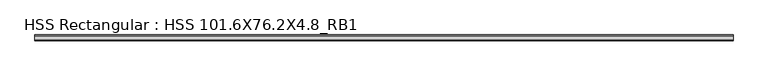
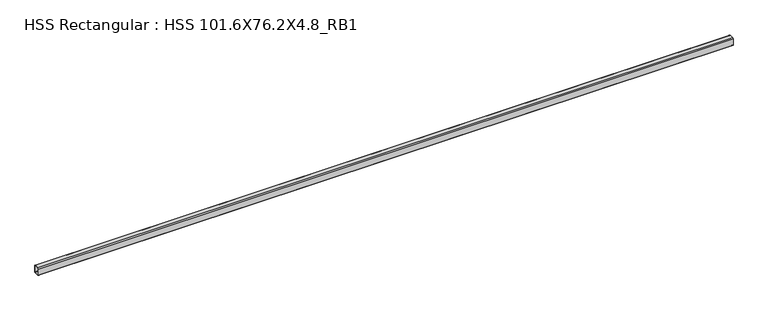
"""IFC4 building model written with IfcOpenShell, lengths in millimetres: beam geometry, HSS Rectangular : HSS 101.6X76.2X4.8_RB1."""

from ifc_helpers import new_model, si_unit, point, frame, frame_2d, origin, place, context, project, spatial, polyline, circle_curve, trimmed, segment, composite_curve, outline, extrude, source, transform, mapped, element, save


def hss_rectangular_hss_101_6x76_2x4_8_rb1_f4add5eb(model_context):
    return source(origin(), model_context, "Body", "SweptSolid", [
        extrude(outline(composite_curve([segment(trimmed(circle_curve(frame_2d((-28.575, 41.275)), 9.525), [point((-38.1, 41.275))], [point((-28.575, 50.8))], False, "CARTESIAN"), True, "CONTINUOUS"), segment(polyline([(-28.575, 50.8), (28.575, 50.8)]), True, "CONTINUOUS"), segment(trimmed(circle_curve(frame_2d((28.575, 41.275)), 9.525), [point((28.575, 50.8))], [point((38.1, 41.275))], False, "CARTESIAN"), True, "CONTINUOUS"), segment(polyline([(38.1, 41.275), (38.1, -41.275)]), True, "CONTINUOUS"), segment(trimmed(circle_curve(frame_2d((28.575, -41.275)), 9.525), [point((38.1, -41.275))], [point((28.575, -50.8))], False, "CARTESIAN"), True, "CONTINUOUS"), segment(polyline([(28.575, -50.8), (-28.575, -50.8)]), True, "CONTINUOUS"), segment(trimmed(circle_curve(frame_2d((-28.575, -41.275)), 9.525), [point((-28.575, -50.8))], [point((-38.1, -41.275))], False, "CARTESIAN"), True, "CONTINUOUS"), segment(polyline([(-38.1, -41.275), (-38.1, 41.275)]), True, "CONTINUOUS")], self_intersect=False), holes=[composite_curve([segment(polyline([(28.575, 46.0375), (-28.575, 46.0375)]), True, "CONTINUOUS"), segment(trimmed(circle_curve(frame_2d((-28.575, 41.275)), 4.7625), [point((-28.575, 46.0375))], [point((-33.3375, 41.275))], True, "CARTESIAN"), True, "CONTINUOUS"), segment(polyline([(-33.3375, 41.275), (-33.3375, -41.275)]), True, "CONTINUOUS"), segment(trimmed(circle_curve(frame_2d((-28.575, -41.275)), 4.7625), [point((-33.3375, -41.275))], [point((-28.575, -46.0375))], True, "CARTESIAN"), True, "CONTINUOUS"), segment(polyline([(-28.575, -46.0375), (28.575, -46.0375)]), True, "CONTINUOUS"), segment(trimmed(circle_curve(frame_2d((28.575, -41.275)), 4.7625), [point((28.575, -46.0375))], [point((33.3375, -41.275))], True, "CARTESIAN"), True, "CONTINUOUS"), segment(polyline([(33.3375, -41.275), (33.3375, 41.275)]), True, "CONTINUOUS"), segment(trimmed(circle_curve(frame_2d((28.575, 41.275)), 4.7625), [point((33.3375, 41.275))], [point((28.575, 46.0375))], True, "CARTESIAN"), True, "CONTINUOUS")], self_intersect=False)]), frame((-7457.3609994, 0.0, 0.0), z_axis=(1.0, 0.0, 0.0), x_axis=(0.0, 1.0, 0.0)), (0.0, 0.0, 1.0), 8995.4609994),
    ])


if __name__ == "__main__":
    model = new_model("IFC4")
    model_context = context("Model", 3, world=origin())
    ifc_project = project(units=[si_unit("LENGTHUNIT", "METRE", prefix="MILLI")], contexts=[model_context])
    site = spatial("IfcSite", under=ifc_project)
    building = spatial("IfcBuilding", under=site)
    placement = place(None, origin())
    hss_rectangular_hss_101_6x76_2x4_8_rb1_shape = hss_rectangular_hss_101_6x76_2x4_8_rb1_f4add5eb(model_context)
    element("IfcBeam", 1, ObjectType="HSS Rectangular : HSS 101.6X76.2X4.8_RB1", at=placement, inside=building, context=model_context, shape_type="MappedRepresentation", body=[
        mapped(hss_rectangular_hss_101_6x76_2x4_8_rb1_shape, transform((0.0, 0.0, 0.0), x_axis=(1.0, 0.0, 0.0), y_axis=(0.0, 1.0, 0.0), z_axis=(0.0, 0.0, 1.0))),
    ])
    save(model, "model.ifc")

# Revit data of these elements
# Type "HSS Rectangular : HSS 101.6X76.2X4.8_RB1"
#   Section Name Key = "HSS 4X3X3/16"
#   Assembly Code = "B10"
#   Width = 7.62 cm
#   Wall Nominal Thickness = 0.4763 cm
#   Wall Design Thickness = 0.442 cm
#   Torsional Moment of Inertia = 260.561 cm⁴
#   Torsional Modulus = 61.2876 cm³
#   Section Area = 14.4516 cm²
#   Plastic Modulus weak axis = 40.3122 cm³
#   Plastic Modulus strong axis = 49.1612 cm³
#   Perimeter = 0.881482 m²/m
#   Outer Fillet = 0.9525 cm
#   Nominal Weight = 12.1285 kgf/m
#   Moment of Inertia weak axis = 131.529 cm⁴
#   Moment of Inertia strong axis = 205.202 cm⁴
#   Inner Fillet = 0.4763 cm
#   Height = 10.16 cm
#   Elastic Modulus weak axis = 34.4128 cm³
#   Elastic Modulus strong axis = 40.476 cm³
#   Centroid Vertical = 5.08 cm
#   Centroid Horizontal = 3.81 cm
#   Length [instance default] = 1524 mm
#   Structural Material [instance default] = Steel ASTM A500, Grade B, Rectangular and Square
#   Principal Axes Angle = 0
# Element 1 (IfcBeam, "HSS Rectangular : HSS 101.6X76.2X4.8_RB1")
#   Structural Material = Steel ASTM A992
#   Materials on its faces: "Steel ASTM A992"
# Materials
#   "Steel ASTM A500, Grade B, Rectangular and Square": class "Metal", colour RGB 199 199 199, transparency 0, Description = "Carbon steel", Cost = 0
#   "Steel ASTM A992": class "Metal", colour RGB 199 199 199, transparency 0, Description = "Structural steel 50ksi", Cost = 0
